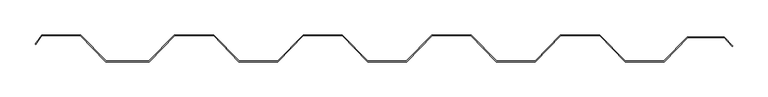
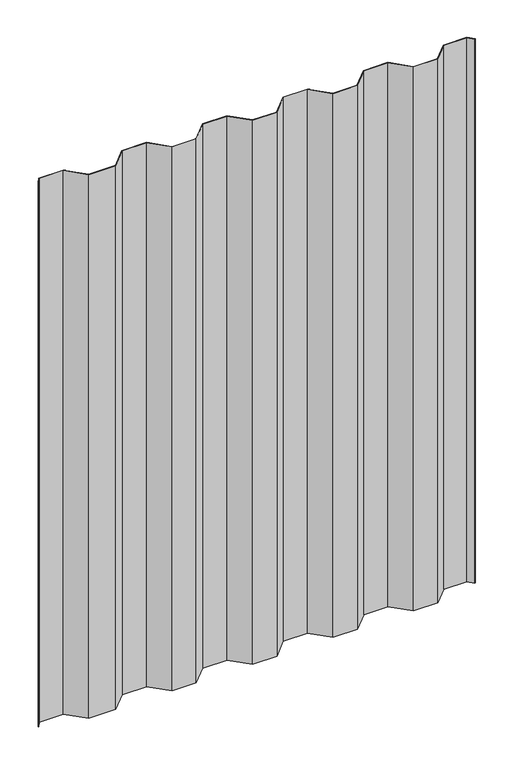
"""IFC4 building model written with IfcOpenShell, lengths in millimetres: proxy geometry, Generic Models 2:Generic Models 2:310765:Generic Models 2:310765 : Generic Models 2:Generic Models 2:310765:58 : Generic Models 2:Generic Models 2:310765:Generic Models 2:310765 : Generic Models 2:Generic Models 2:310765:300385."""

from ifc_helpers import new_model, si_unit, frame, origin, place, context, project, spatial, polyline, outline, extrude, source, transform, mapped, element, save


def generic_models_89070665(model_context):
    return source(origin(), model_context, "Body", "SweptSolid", [
        extrude(outline(polyline([(600921.7908534, -566348.0253389), (600933.6465997, -566361.1334099), (600933.0846279, -566361.6953817), (600921.4385161, -566348.8190889), (600869.5321621, -566348.8190889), (600835.9001773, -566383.3771761), (600780.7206174, -566383.3771761), (600744.5584258, -566346.0709261), (600689.1833002, -566346.0709261), (600653.0211085, -566383.3771761), (600597.8406174, -566383.3771761), (600561.6784258, -566346.0709261), (600506.3033002, -566346.0709261), (600470.1411085, -566383.3771761), (600414.9606174, -566383.3771761), (600378.7984258, -566346.0709261), (600323.4233002, -566346.0709261), (600287.2611085, -566383.3771761), (600232.0806174, -566383.3771761), (600195.9184258, -566346.0709261), (600140.5433002, -566346.0709261), (600104.3811085, -566383.3771761), (600042.8506174, -566383.3771761), (600006.6884258, -566346.0709261), (599952.159863, -566346.0709261), (599943.2184948, -566358.8405234), (599942.5682928, -566358.3852471), (599951.746663, -566345.2771761), (600007.0244713, -566345.2771761), (600043.186663, -566382.5834261), (600104.045063, -566382.5834261), (600140.2072546, -566345.2771761), (600196.2544713, -566345.2771761), (600232.416663, -566382.5834261), (600286.925063, -566382.5834261), (600323.0872546, -566345.2771761), (600379.1344713, -566345.2771761), (600415.296663, -566382.5834261), (600469.805063, -566382.5834261), (600505.9672546, -566345.2771761), (600562.0144713, -566345.2771761), (600598.176663, -566382.5834261), (600652.685063, -566382.5834261), (600688.8472546, -566345.2771761), (600744.8944713, -566345.2771761), (600781.056663, -566382.5834261), (600835.565063, -566382.5834261), (600869.1970477, -566348.0253389), (600921.7908534, -566348.0253389)])), frame((0.0, 0.0, 4656.1018378), z_axis=(0.0, 0.0, 1.0), x_axis=(1.0, 0.0, 0.0)), (0.0, 0.0, 1.0), 1305.250742),
    ])


if __name__ == "__main__":
    model = new_model("IFC4")
    model_context = context("Model", 3, world=origin())
    ifc_project = project(units=[si_unit("LENGTHUNIT", "METRE", prefix="MILLI")], contexts=[model_context])
    site = spatial("IfcSite", under=ifc_project)
    building = spatial("IfcBuilding", under=site)
    placement = place(None, origin())
    generic_models_shape = generic_models_89070665(model_context)
    element("IfcBuildingElementProxy", 1, Name="Generic Models 2:Generic Models 2:310765:Generic Models 2:310765 : Generic Models 2:Generic Models 2:310765:58 : Generic Models 2:Generic Models 2:310765:Generic Models 2:310765 : Generic Models 2:Generic Models 2:310765:300385", ObjectType="Generic Models 2:Generic Models 2:310765:Generic Models 2:310765 : Generic Models 2:Generic Models 2:310765:58 : Generic Models 2:Generic Models 2:310765:Generic Models 2:310765 : Generic Models 2:Generic Models 2:310765:300385", at=placement, inside=building, context=model_context, shape_type="MappedRepresentation", body=[
        mapped(generic_models_shape, transform((0.0, 0.0, 0.0), x_axis=(1.0, 0.0, 0.0), y_axis=(0.0, 1.0, 0.0), z_axis=(0.0, 0.0, 1.0))),
    ])
    save(model, "model.ifc")

# Revit data of these elements
# Type "Generic Models 2:Generic Models 2:310765:Generic Models 2:310765 : Generic Models 2:Generic Models 2:310765:58 : Generic Models 2:Generic Models 2:310765:Generic Models 2:310765 : Generic Models 2:Generic Models 2:310765:300385"
#   NameOverride = "Generic Models 2:Generic Models 2:310765:Generic Models 2:310765 : Generic Models 2:Generic Models 2:310765:300385"
#   ObjectTypeOverride = "Generic Models 2:310765 : Generic Models 2:Generic Models 2:310765"
#   Reference = "Generic Models 2"
#   Tag = "300385"
# Element 1 (IfcBuildingElementProxy, "Generic Models 2:Generic Models 2:310765:Generic Models 2:310765 : Generic Models 2:Generic Models 2:310765:58 : Generic Models 2:Generic Models 2:310765:Generic Models 2:310765 : Generic Models 2:Generic Models 2:310765:300385")
#   Materials on its faces: "THERMAL BROKEN ALUMINUM STOREFRONT FOR POLYCARBONATE"
# Materials
#   "THERMAL BROKEN ALUMINUM STOREFRONT FOR POLYCARBONATE": class "Unassigned", colour RGB 244 244 244, transparency 0, Keynote = "M07611300.01", Cost = 0
